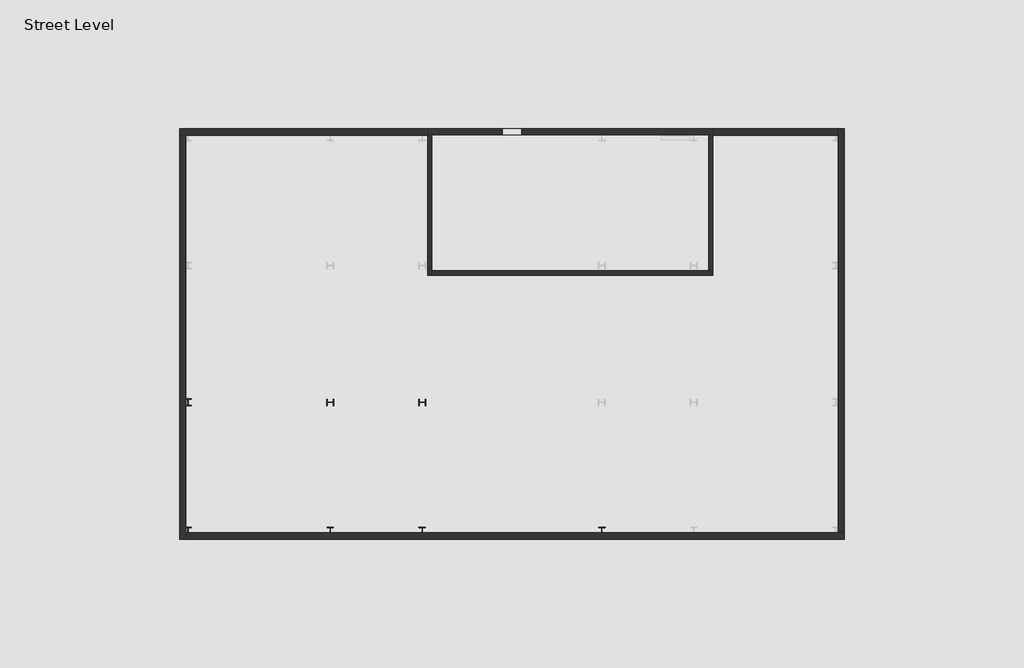
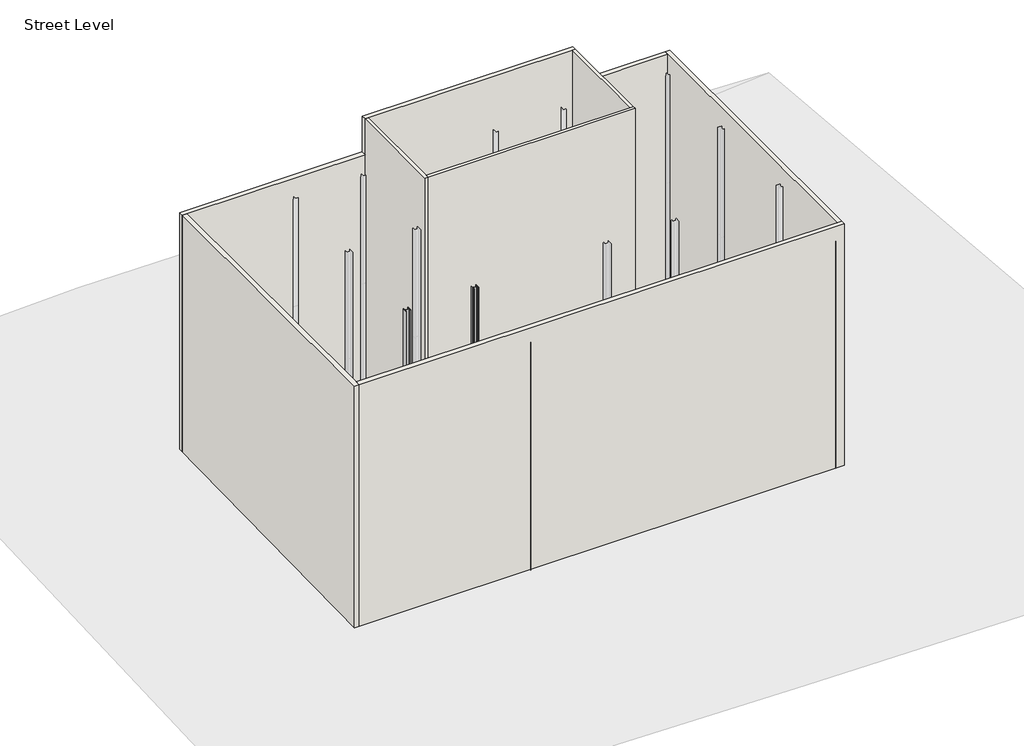
# One storey, part 1 of 3: 9 walls, 7 columns.
"""IFC4 building model written with IfcOpenShell, lengths in millimetres."""

import ifcopenshell
import ifcopenshell.guid

model = None  # the IFC model being written
_history = None  # IfcOwnerHistory: only IFC2X3 demands one
_inside = {}  # id of a spatial element -> (the spatial element, [elements in it])
_under = {}  # id of a project, library or spatial element -> (it, [spatial elements below it])
_declared = {}  # id of a project -> (the project, [libraries it declares])
_typed = {}  # id of a type object -> (the type object, [elements of that type])
_made_of = {}  # id of a material, layer set ... -> (it, [elements and type objects made of it])


def new_model(schema):
    """Start an empty IFC model of exactly this schema.

    Asked for "IFC4X3", IfcOpenShell would pick the latest addendum, in which some entities
    have other attributes; the version numbers below select the first issue.
    IFC2X3 requires an IfcOwnerHistory on every rooted entity: one is made here for all.
    """
    global model, _history
    if schema == "IFC4X3":
        model = ifcopenshell.file(schema_version=(4, 3, 0, 0))
    else:
        model = ifcopenshell.file(schema=schema)
    _inside.clear()
    _under.clear()
    _declared.clear()
    _typed.clear()
    _made_of.clear()
    _history = None
    if model.schema == "IFC2X3":
        org = make("IfcOrganization", Name="unknown")
        user = make(
            "IfcPersonAndOrganization",
            ThePerson=make("IfcPerson", FamilyName="unknown"),
            TheOrganization=org,
        )
        app = make(
            "IfcApplication",
            ApplicationDeveloper=org,
            Version="unknown",
            ApplicationFullName="unknown",
            ApplicationIdentifier="unknown",
        )
        _history = make(
            "IfcOwnerHistory",
            OwningUser=user,
            OwningApplication=app,
            ChangeAction="ADDED",
            CreationDate=0,
        )
    return model


def make(cls, **values):
    """One entity of the class cls with the attributes given. An attribute that is None is left unset."""
    return model.create_entity(
        cls, **{name: value for name, value in values.items() if value is not None}
    )


def rooted(cls, **values):
    """An entity with a GlobalId (a new one), such as an element, a storey or a relation."""
    return make(cls, GlobalId=ifcopenshell.guid.new(), OwnerHistory=_history, **values)


def si_unit(unit_type, name, prefix=None):
    """IfcSIUnit, for example si_unit("LENGTHUNIT", "METRE", prefix="MILLI")."""
    return make("IfcSIUnit", UnitType=unit_type, Prefix=prefix, Name=name)


def assignment(units):
    """IfcUnitAssignment: the units of a project."""
    return None if units is None else make("IfcUnitAssignment", Units=units)


def point(xyz):
    """IfcCartesianPoint."""
    return None if xyz is None else make("IfcCartesianPoint", Coordinates=xyz)


def direction(xyz):
    """IfcDirection."""
    return None if xyz is None else make("IfcDirection", DirectionRatios=xyz)


def frame(location, z_axis=None, x_axis=None):
    """IfcAxis2Placement3D, a coordinate frame: its origin and axes. An axis left out is left unset."""
    return make(
        "IfcAxis2Placement3D",
        Location=point(location),
        Axis=direction(z_axis),
        RefDirection=direction(x_axis),
    )


def frame_2d(location, x_axis=None):
    """IfcAxis2Placement2D, a coordinate frame in the plane: its origin and x axis."""
    return make(
        "IfcAxis2Placement2D", Location=point(location), RefDirection=direction(x_axis)
    )


def origin():
    """The frame at (0, 0, 0) with its axes left unset."""
    return frame((0.0, 0.0, 0.0))


def place(relative_to, where):
    """IfcLocalPlacement: puts the frame where relative to a parent placement (None: the world)."""
    return make(
        "IfcLocalPlacement", PlacementRelTo=relative_to, RelativePlacement=where
    )


def context(
    kind, dimensions, precision=None, world=None, true_north=None, identifier=None
):
    """IfcGeometricRepresentationContext, for example the 3D "Model" context."""
    return make(
        "IfcGeometricRepresentationContext",
        ContextIdentifier=identifier,
        ContextType=kind,
        CoordinateSpaceDimension=dimensions,
        Precision=precision,
        WorldCoordinateSystem=world,
        TrueNorth=true_north,
    )


def project(units=None, contexts=None):
    """IfcProject with its units and contexts."""
    return rooted(
        "IfcProject",
        Name="project",
        RepresentationContexts=contexts,
        UnitsInContext=assignment(units),
    )


def spatial(cls, under=None, at=None, **own):
    """A site, building, storey or space (cls), placed at a placement, below another one or the project."""
    s = rooted(cls, ObjectPlacement=at, **own)
    if under is not None:
        _under.setdefault(under.id(), (under, []))[1].append(s)
    return s


def polyline(points):
    """IfcPolyline through the points."""
    return make("IfcPolyline", Points=[point(p) for p in points])


def circle_curve(where, radius):
    """IfcCircle in the frame where."""
    return make("IfcCircle", Position=where, Radius=radius)


def trimmed(basis, trim1, trim2, sense, master):
    """IfcTrimmedCurve: the piece of a basis curve between two trims."""
    return make(
        "IfcTrimmedCurve",
        BasisCurve=basis,
        Trim1=trim1,
        Trim2=trim2,
        SenseAgreement=sense,
        MasterRepresentation=master,
    )


def segment(curve, same_sense, transition):
    """IfcCompositeCurveSegment."""
    return make(
        "IfcCompositeCurveSegment",
        Transition=transition,
        SameSense=same_sense,
        ParentCurve=curve,
    )


def composite_curve(segments, self_intersect=None):
    """IfcCompositeCurve: segments joined end to end."""
    return make("IfcCompositeCurve", Segments=segments, SelfIntersect=self_intersect)


def outline(outer, holes=None, kind="AREA"):
    """IfcArbitraryClosedProfileDef: a profile drawn as a closed curve; with holes, ...WithVoids."""
    if holes is None:
        return make("IfcArbitraryClosedProfileDef", ProfileType=kind, OuterCurve=outer)
    return make(
        "IfcArbitraryProfileDefWithVoids",
        ProfileType=kind,
        OuterCurve=outer,
        InnerCurves=holes,
    )


def extrude(swept, where, along, depth):
    """IfcExtrudedAreaSolid: the profile swept, set in the frame where, extruded along a direction by depth."""
    return make(
        "IfcExtrudedAreaSolid",
        SweptArea=swept,
        Position=where,
        ExtrudedDirection=direction(along),
        Depth=depth,
    )


def faces_of(points, faces, orient=None, outer=None):
    """IfcFace entities. A face is a list of loops; a loop is a list of indices into points, from 0.

    orient and outer hold one flag for each loop. By default every Orientation is true, the
    first loop of a face is its IfcFaceOuterBound and the others are IfcFaceBound.
    """
    made = []
    for i, loops in enumerate(faces):
        bounds = []
        for j, loop in enumerate(loops):
            is_outer = j == 0 if outer is None else outer[i][j]
            bounds.append(
                make(
                    "IfcFaceOuterBound" if is_outer else "IfcFaceBound",
                    Bound=make("IfcPolyLoop", Polygon=[points[k] for k in loop]),
                    Orientation=True if orient is None else orient[i][j],
                )
            )
        made.append(make("IfcFace", Bounds=bounds))
    return made


def faceted_brep(points, faces, orient=None, outer=None, voids=None):
    """IfcFacetedBrep: a solid bounded by flat faces; with voids (closed shells), ...WithVoids."""
    shared = [point(p) for p in points]
    hull = make("IfcClosedShell", CfsFaces=faces_of(shared, faces, orient, outer))
    if voids is None:
        return make("IfcFacetedBrep", Outer=hull)
    return make(
        "IfcFacetedBrepWithVoids",
        Outer=hull,
        Voids=[
            make(cls, CfsFaces=faces_of(shared, fs, o, b)) for cls, fs, o, b in voids
        ],
    )


def shape(context_of_items, identifier, shape_type, items):
    """IfcShapeRepresentation: the items that make up one representation, for example the "Body"."""
    return make(
        "IfcShapeRepresentation",
        ContextOfItems=context_of_items,
        RepresentationIdentifier=identifier,
        RepresentationType=shape_type,
        Items=items,
    )


def made_of(thing, what):
    """Note that an element or type object is made of a material, layer set ...; save() writes the relation."""
    if what is not None:
        _made_of.setdefault(what.id(), (what, []))[1].append(thing)
    return thing


def element(
    cls,
    number,
    at=None,
    inside=None,
    cuts=None,
    type_object=None,
    material=None,
    context=None,
    identifier="Body",
    shape_type=None,
    held_by="IfcProductDefinitionShape",
    body=None,
    shapes=None,
    **own,
):
    """One element of the class cls, such as IfcWall. Its Tag is "e" and its number.

    at: its placement. inside: the storey or other place that contains it. cuts: it is an
    opening in that element (IfcRelVoidsElement). A single representation is given by context,
    identifier, shape_type and body (its items); several are given by shapes. held_by: the class
    of the entity that holds the representations. save() writes the other relations.
    """
    e = rooted(cls, Tag="e%d" % number, ObjectPlacement=at, **own)
    if body is not None:
        shapes = [shape(context, identifier, shape_type, body)]
    if shapes is not None:
        e.Representation = make(held_by, Representations=shapes)
    if inside is not None:
        _inside.setdefault(inside.id(), (inside, []))[1].append(e)
    if cuts is not None:
        rooted(
            "IfcRelVoidsElement", RelatingBuildingElement=cuts, RelatedOpeningElement=e
        )
    if type_object is not None:
        _typed.setdefault(type_object.id(), (type_object, []))[1].append(e)
    return made_of(e, material)


def aggregate(whole, parts):
    """IfcRelAggregates: a whole, such as a stair, and the parts it consists of."""
    return rooted("IfcRelAggregates", RelatingObject=whole, RelatedObjects=parts)


def save(model, path):
    """Write the relations noted so far, then the file.

    IfcRelAggregates (storeys below a building ...), IfcRelContainedInSpatialStructure (elements
    in a storey), IfcRelDefinesByType, IfcRelAssociatesMaterial and IfcRelDeclares: one each for
    every whole, place, type object, material and project.
    """
    for whole, parts in _under.values():
        aggregate(whole, parts)
    for where, things in _inside.values():
        rooted(
            "IfcRelContainedInSpatialStructure",
            RelatedElements=things,
            RelatingStructure=where,
        )
    for kind, things in _typed.values():
        rooted("IfcRelDefinesByType", RelatedObjects=things, RelatingType=kind)
    for what, things in _made_of.values():
        rooted("IfcRelAssociatesMaterial", RelatedObjects=things, RelatingMaterial=what)
    for by, libraries in _declared.values():
        rooted("IfcRelDeclares", RelatingContext=by, RelatedDefinitions=libraries)
    model.write(path)


model = new_model("IFC4")

# Units and contexts
model_context = context("Model", 3, world=origin())
ifc_project = project(units=[si_unit("LENGTHUNIT", "METRE", prefix="MILLI")], contexts=[model_context])

# Site, building, storey
site = spatial("IfcSite", under=ifc_project)
building = spatial("IfcBuilding", under=site)
storey = spatial("IfcBuildingStorey", under=building, Name="Street Level", Elevation=-914.4)

# Columns
placement = place(None, origin())
element("IfcColumn", 1, ObjectType="W-Wide Flange-Column : W12X87", at=placement, inside=storey, context=model_context, shape_type="SweptSolid", body=[
    extrude(outline(composite_curve([segment(polyline([(-9643.0622732, -3562.1684696), (-9663.6362732, -3562.1684696), (-9663.6362732, -3437.3274696)]), True, "CONTINUOUS"), segment(trimmed(circle_curve(frame_2d((-9685.9247732, -3437.3274696)), 22.2885), [point((-9663.6362732, -3437.3274696))], [point((-9685.9247732, -3415.0389696))], True, "CARTESIAN"), True, "CONTINUOUS"), segment(polyline([(-9685.9247732, -3415.0389696), (-9917.6997732, -3415.0389696)]), True, "CONTINUOUS"), segment(trimmed(circle_curve(frame_2d((-9917.6997732, -3437.3274696)), 22.2885), [point((-9917.6997732, -3415.0389696))], [point((-9939.9882732, -3437.3274696))], True, "CARTESIAN"), True, "CONTINUOUS"), segment(polyline([(-9939.9882732, -3437.3274696), (-9939.9882732, -3562.1684696), (-9960.5622732, -3562.1684696), (-9960.5622732, -3254.8284696), (-9939.9882732, -3254.8284696), (-9939.9882732, -3379.6694696)]), True, "CONTINUOUS"), segment(trimmed(circle_curve(frame_2d((-9917.6997732, -3379.6694696)), 22.2885), [point((-9939.9882732, -3379.6694696))], [point((-9917.6997732, -3401.9579696))], True, "CARTESIAN"), True, "CONTINUOUS"), segment(polyline([(-9917.6997732, -3401.9579696), (-9685.9247732, -3401.9579696)]), True, "CONTINUOUS"), segment(trimmed(circle_curve(frame_2d((-9685.9247732, -3379.6694696)), 22.2885), [point((-9685.9247732, -3401.9579696))], [point((-9663.6362732, -3379.6694696))], True, "CARTESIAN"), True, "CONTINUOUS"), segment(polyline([(-9663.6362732, -3379.6694696), (-9663.6362732, -3254.8284696), (-9643.0622732, -3254.8284696), (-9643.0622732, -3562.1684696)]), True, "CONTINUOUS")], self_intersect=False)), frame((0.0, 0.0, 7315.2), z_axis=(0.0, 0.0, 1.0), x_axis=(1.0, 0.0, 0.0)), (0.0, 0.0, 1.0), 7315.2),
    extrude(outline(composite_curve([segment(polyline([(-9643.0622732, -3562.1684696), (-9663.6362732, -3562.1684696), (-9663.6362732, -3437.3274696)]), True, "CONTINUOUS"), segment(trimmed(circle_curve(frame_2d((-9685.9247732, -3437.3274696)), 22.2885), [point((-9663.6362732, -3437.3274696))], [point((-9685.9247732, -3415.0389696))], True, "CARTESIAN"), True, "CONTINUOUS"), segment(polyline([(-9685.9247732, -3415.0389696), (-9917.6997732, -3415.0389696)]), True, "CONTINUOUS"), segment(trimmed(circle_curve(frame_2d((-9917.6997732, -3437.3274696)), 22.2885), [point((-9917.6997732, -3415.0389696))], [point((-9939.9882732, -3437.3274696))], True, "CARTESIAN"), True, "CONTINUOUS"), segment(polyline([(-9939.9882732, -3437.3274696), (-9939.9882732, -3562.1684696), (-9960.5622732, -3562.1684696), (-9960.5622732, -3254.8284696), (-9939.9882732, -3254.8284696), (-9939.9882732, -3379.6694696)]), True, "CONTINUOUS"), segment(trimmed(circle_curve(frame_2d((-9917.6997732, -3379.6694696)), 22.2885), [point((-9939.9882732, -3379.6694696))], [point((-9917.6997732, -3401.9579696))], True, "CARTESIAN"), True, "CONTINUOUS"), segment(polyline([(-9917.6997732, -3401.9579696), (-9685.9247732, -3401.9579696)]), True, "CONTINUOUS"), segment(trimmed(circle_curve(frame_2d((-9685.9247732, -3379.6694696)), 22.2885), [point((-9685.9247732, -3401.9579696))], [point((-9663.6362732, -3379.6694696))], True, "CARTESIAN"), True, "CONTINUOUS"), segment(polyline([(-9663.6362732, -3379.6694696), (-9663.6362732, -3254.8284696), (-9643.0622732, -3254.8284696), (-9643.0622732, -3562.1684696)]), True, "CONTINUOUS")], self_intersect=False)), frame((0.0, 0.0, -914.4), z_axis=(0.0, 0.0, 1.0), x_axis=(1.0, 0.0, 0.0)), (0.0, 0.0, 1.0), 8229.6),
])
element("IfcColumn", 2, ObjectType="W-Wide Flange-Column : W12X87", at=placement, inside=storey, context=model_context, shape_type="SweptSolid", body=[
    extrude(outline(composite_curve([segment(polyline([(-5274.2622732, -3562.1684696), (-5294.8362732, -3562.1684696), (-5294.8362732, -3437.3274696)]), True, "CONTINUOUS"), segment(trimmed(circle_curve(frame_2d((-5317.1247732, -3437.3274696)), 22.2885), [point((-5294.8362732, -3437.3274696))], [point((-5317.1247732, -3415.0389696))], True, "CARTESIAN"), True, "CONTINUOUS"), segment(polyline([(-5317.1247732, -3415.0389696), (-5548.8997732, -3415.0389696)]), True, "CONTINUOUS"), segment(trimmed(circle_curve(frame_2d((-5548.8997732, -3437.3274696)), 22.2885), [point((-5548.8997732, -3415.0389696))], [point((-5571.1882732, -3437.3274696))], True, "CARTESIAN"), True, "CONTINUOUS"), segment(polyline([(-5571.1882732, -3437.3274696), (-5571.1882732, -3562.1684696), (-5591.7622732, -3562.1684696), (-5591.7622732, -3254.8284696), (-5571.1882732, -3254.8284696), (-5571.1882732, -3379.6694696)]), True, "CONTINUOUS"), segment(trimmed(circle_curve(frame_2d((-5548.8997732, -3379.6694696)), 22.2885), [point((-5571.1882732, -3379.6694696))], [point((-5548.8997732, -3401.9579696))], True, "CARTESIAN"), True, "CONTINUOUS"), segment(polyline([(-5548.8997732, -3401.9579696), (-5317.1247732, -3401.9579696)]), True, "CONTINUOUS"), segment(trimmed(circle_curve(frame_2d((-5317.1247732, -3379.6694696)), 22.2885), [point((-5317.1247732, -3401.9579696))], [point((-5294.8362732, -3379.6694696))], True, "CARTESIAN"), True, "CONTINUOUS"), segment(polyline([(-5294.8362732, -3379.6694696), (-5294.8362732, -3254.8284696), (-5274.2622732, -3254.8284696), (-5274.2622732, -3562.1684696)]), True, "CONTINUOUS")], self_intersect=False)), frame((0.0, 0.0, 7315.2), z_axis=(0.0, 0.0, 1.0), x_axis=(1.0, 0.0, 0.0)), (0.0, 0.0, 1.0), 7315.2),
    extrude(outline(composite_curve([segment(polyline([(-5274.2622732, -3562.1684696), (-5294.8362732, -3562.1684696), (-5294.8362732, -3437.3274696)]), True, "CONTINUOUS"), segment(trimmed(circle_curve(frame_2d((-5317.1247732, -3437.3274696)), 22.2885), [point((-5294.8362732, -3437.3274696))], [point((-5317.1247732, -3415.0389696))], True, "CARTESIAN"), True, "CONTINUOUS"), segment(polyline([(-5317.1247732, -3415.0389696), (-5548.8997732, -3415.0389696)]), True, "CONTINUOUS"), segment(trimmed(circle_curve(frame_2d((-5548.8997732, -3437.3274696)), 22.2885), [point((-5548.8997732, -3415.0389696))], [point((-5571.1882732, -3437.3274696))], True, "CARTESIAN"), True, "CONTINUOUS"), segment(polyline([(-5571.1882732, -3437.3274696), (-5571.1882732, -3562.1684696), (-5591.7622732, -3562.1684696), (-5591.7622732, -3254.8284696), (-5571.1882732, -3254.8284696), (-5571.1882732, -3379.6694696)]), True, "CONTINUOUS"), segment(trimmed(circle_curve(frame_2d((-5548.8997732, -3379.6694696)), 22.2885), [point((-5571.1882732, -3379.6694696))], [point((-5548.8997732, -3401.9579696))], True, "CARTESIAN"), True, "CONTINUOUS"), segment(polyline([(-5548.8997732, -3401.9579696), (-5317.1247732, -3401.9579696)]), True, "CONTINUOUS"), segment(trimmed(circle_curve(frame_2d((-5317.1247732, -3379.6694696)), 22.2885), [point((-5317.1247732, -3401.9579696))], [point((-5294.8362732, -3379.6694696))], True, "CARTESIAN"), True, "CONTINUOUS"), segment(polyline([(-5294.8362732, -3379.6694696), (-5294.8362732, -3254.8284696), (-5274.2622732, -3254.8284696), (-5274.2622732, -3562.1684696)]), True, "CONTINUOUS")], self_intersect=False)), frame((0.0, 0.0, -914.4), z_axis=(0.0, 0.0, 1.0), x_axis=(1.0, 0.0, 0.0)), (0.0, 0.0, 1.0), 8229.6),
])
element("IfcColumn", 3, ObjectType="W-Wide Flange-Column : W12X87", at=placement, inside=storey, context=model_context, shape_type="SweptSolid", body=[
    extrude(outline(composite_curve([segment(polyline([(3255.0577268, -9345.7484696), (3255.0577268, -9366.3224696), (3130.2167268, -9366.3224696)]), True, "CONTINUOUS"), segment(trimmed(circle_curve(frame_2d((3130.2167268, -9388.6109696)), 22.2885), [point((3130.2167268, -9366.3224696))], [point((3107.9282268, -9388.6109696))], True, "CARTESIAN"), True, "CONTINUOUS"), segment(polyline([(3107.9282268, -9388.6109696), (3107.9282268, -9620.3859696)]), True, "CONTINUOUS"), segment(trimmed(circle_curve(frame_2d((3130.2167268, -9620.3859696)), 22.2885), [point((3107.9282268, -9620.3859696))], [point((3130.2167268, -9642.6744696))], True, "CARTESIAN"), True, "CONTINUOUS"), segment(polyline([(3130.2167268, -9642.6744696), (3255.0577268, -9642.6744696), (3255.0577268, -9663.2484696), (2947.7177268, -9663.2484696), (2947.7177268, -9642.6744696), (3072.5587268, -9642.6744696)]), True, "CONTINUOUS"), segment(trimmed(circle_curve(frame_2d((3072.5587268, -9620.3859696)), 22.2885), [point((3072.5587268, -9642.6744696))], [point((3094.8472268, -9620.3859696))], True, "CARTESIAN"), True, "CONTINUOUS"), segment(polyline([(3094.8472268, -9620.3859696), (3094.8472268, -9388.6109696)]), True, "CONTINUOUS"), segment(trimmed(circle_curve(frame_2d((3072.5587268, -9388.6109696)), 22.2885), [point((3094.8472268, -9388.6109696))], [point((3072.5587268, -9366.3224696))], True, "CARTESIAN"), True, "CONTINUOUS"), segment(polyline([(3072.5587268, -9366.3224696), (2947.7177268, -9366.3224696), (2947.7177268, -9345.7484696), (3255.0577268, -9345.7484696)]), True, "CONTINUOUS")], self_intersect=False)), frame((0.0, 0.0, 7315.2), z_axis=(0.0, 0.0, 1.0), x_axis=(1.0, 0.0, 0.0)), (0.0, 0.0, 1.0), 7315.2),
    extrude(outline(composite_curve([segment(polyline([(3255.0577268, -9345.7484696), (3255.0577268, -9366.3224696), (3130.2167268, -9366.3224696)]), True, "CONTINUOUS"), segment(trimmed(circle_curve(frame_2d((3130.2167268, -9388.6109696)), 22.2885), [point((3130.2167268, -9366.3224696))], [point((3107.9282268, -9388.6109696))], True, "CARTESIAN"), True, "CONTINUOUS"), segment(polyline([(3107.9282268, -9388.6109696), (3107.9282268, -9620.3859696)]), True, "CONTINUOUS"), segment(trimmed(circle_curve(frame_2d((3130.2167268, -9620.3859696)), 22.2885), [point((3107.9282268, -9620.3859696))], [point((3130.2167268, -9642.6744696))], True, "CARTESIAN"), True, "CONTINUOUS"), segment(polyline([(3130.2167268, -9642.6744696), (3255.0577268, -9642.6744696), (3255.0577268, -9663.2484696), (2947.7177268, -9663.2484696), (2947.7177268, -9642.6744696), (3072.5587268, -9642.6744696)]), True, "CONTINUOUS"), segment(trimmed(circle_curve(frame_2d((3072.5587268, -9620.3859696)), 22.2885), [point((3072.5587268, -9642.6744696))], [point((3094.8472268, -9620.3859696))], True, "CARTESIAN"), True, "CONTINUOUS"), segment(polyline([(3094.8472268, -9620.3859696), (3094.8472268, -9388.6109696)]), True, "CONTINUOUS"), segment(trimmed(circle_curve(frame_2d((3072.5587268, -9388.6109696)), 22.2885), [point((3094.8472268, -9388.6109696))], [point((3072.5587268, -9366.3224696))], True, "CARTESIAN"), True, "CONTINUOUS"), segment(polyline([(3072.5587268, -9366.3224696), (2947.7177268, -9366.3224696), (2947.7177268, -9345.7484696), (3255.0577268, -9345.7484696)]), True, "CONTINUOUS")], self_intersect=False)), frame((0.0, 0.0, -914.4), z_axis=(0.0, 0.0, 1.0), x_axis=(1.0, 0.0, 0.0)), (0.0, 0.0, 1.0), 8229.6),
])
element("IfcColumn", 4, ObjectType="W-Wide Flange-Column : W12X87", at=placement, inside=storey, context=model_context, shape_type="SweptSolid", body=[
    extrude(outline(composite_curve([segment(polyline([(-5279.3422732, -9345.7484696), (-5279.3422732, -9366.3224696), (-5404.1832732, -9366.3224696)]), True, "CONTINUOUS"), segment(trimmed(circle_curve(frame_2d((-5404.1832732, -9388.6109696)), 22.2885), [point((-5404.1832732, -9366.3224696))], [point((-5426.4717732, -9388.6109696))], True, "CARTESIAN"), True, "CONTINUOUS"), segment(polyline([(-5426.4717732, -9388.6109696), (-5426.4717732, -9620.3859696)]), True, "CONTINUOUS"), segment(trimmed(circle_curve(frame_2d((-5404.1832732, -9620.3859696)), 22.2885), [point((-5426.4717732, -9620.3859696))], [point((-5404.1832732, -9642.6744696))], True, "CARTESIAN"), True, "CONTINUOUS"), segment(polyline([(-5404.1832732, -9642.6744696), (-5279.3422732, -9642.6744696), (-5279.3422732, -9663.2484696), (-5586.6822732, -9663.2484696), (-5586.6822732, -9642.6744696), (-5461.8412732, -9642.6744696)]), True, "CONTINUOUS"), segment(trimmed(circle_curve(frame_2d((-5461.8412732, -9620.3859696)), 22.2885), [point((-5461.8412732, -9642.6744696))], [point((-5439.5527732, -9620.3859696))], True, "CARTESIAN"), True, "CONTINUOUS"), segment(polyline([(-5439.5527732, -9620.3859696), (-5439.5527732, -9388.6109696)]), True, "CONTINUOUS"), segment(trimmed(circle_curve(frame_2d((-5461.8412732, -9388.6109696)), 22.2885), [point((-5439.5527732, -9388.6109696))], [point((-5461.8412732, -9366.3224696))], True, "CARTESIAN"), True, "CONTINUOUS"), segment(polyline([(-5461.8412732, -9366.3224696), (-5586.6822732, -9366.3224696), (-5586.6822732, -9345.7484696), (-5279.3422732, -9345.7484696)]), True, "CONTINUOUS")], self_intersect=False)), frame((0.0, 0.0, 7315.2), z_axis=(0.0, 0.0, 1.0), x_axis=(1.0, 0.0, 0.0)), (0.0, 0.0, 1.0), 7315.2),
    extrude(outline(composite_curve([segment(polyline([(-5279.3422732, -9345.7484696), (-5279.3422732, -9366.3224696), (-5404.1832732, -9366.3224696)]), True, "CONTINUOUS"), segment(trimmed(circle_curve(frame_2d((-5404.1832732, -9388.6109696)), 22.2885), [point((-5404.1832732, -9366.3224696))], [point((-5426.4717732, -9388.6109696))], True, "CARTESIAN"), True, "CONTINUOUS"), segment(polyline([(-5426.4717732, -9388.6109696), (-5426.4717732, -9620.3859696)]), True, "CONTINUOUS"), segment(trimmed(circle_curve(frame_2d((-5404.1832732, -9620.3859696)), 22.2885), [point((-5426.4717732, -9620.3859696))], [point((-5404.1832732, -9642.6744696))], True, "CARTESIAN"), True, "CONTINUOUS"), segment(polyline([(-5404.1832732, -9642.6744696), (-5279.3422732, -9642.6744696), (-5279.3422732, -9663.2484696), (-5586.6822732, -9663.2484696), (-5586.6822732, -9642.6744696), (-5461.8412732, -9642.6744696)]), True, "CONTINUOUS"), segment(trimmed(circle_curve(frame_2d((-5461.8412732, -9620.3859696)), 22.2885), [point((-5461.8412732, -9642.6744696))], [point((-5439.5527732, -9620.3859696))], True, "CARTESIAN"), True, "CONTINUOUS"), segment(polyline([(-5439.5527732, -9620.3859696), (-5439.5527732, -9388.6109696)]), True, "CONTINUOUS"), segment(trimmed(circle_curve(frame_2d((-5461.8412732, -9388.6109696)), 22.2885), [point((-5439.5527732, -9388.6109696))], [point((-5461.8412732, -9366.3224696))], True, "CARTESIAN"), True, "CONTINUOUS"), segment(polyline([(-5461.8412732, -9366.3224696), (-5586.6822732, -9366.3224696), (-5586.6822732, -9345.7484696), (-5279.3422732, -9345.7484696)]), True, "CONTINUOUS")], self_intersect=False)), frame((0.0, 0.0, -914.4), z_axis=(0.0, 0.0, 1.0), x_axis=(1.0, 0.0, 0.0)), (0.0, 0.0, 1.0), 8229.6),
])
element("IfcColumn", 5, ObjectType="W-Wide Flange-Column : W12X87", at=placement, inside=storey, context=model_context, shape_type="SweptSolid", body=[
    extrude(outline(composite_curve([segment(polyline([(-9648.1422732, -9345.7484696), (-9648.1422732, -9366.3224696), (-9772.9832732, -9366.3224696)]), True, "CONTINUOUS"), segment(trimmed(circle_curve(frame_2d((-9772.9832732, -9388.6109696)), 22.2885), [point((-9772.9832732, -9366.3224696))], [point((-9795.2717732, -9388.6109696))], True, "CARTESIAN"), True, "CONTINUOUS"), segment(polyline([(-9795.2717732, -9388.6109696), (-9795.2717732, -9620.3859696)]), True, "CONTINUOUS"), segment(trimmed(circle_curve(frame_2d((-9772.9832732, -9620.3859696)), 22.2885), [point((-9795.2717732, -9620.3859696))], [point((-9772.9832732, -9642.6744696))], True, "CARTESIAN"), True, "CONTINUOUS"), segment(polyline([(-9772.9832732, -9642.6744696), (-9648.1422732, -9642.6744696), (-9648.1422732, -9663.2484696), (-9955.4822732, -9663.2484696), (-9955.4822732, -9642.6744696), (-9830.6412732, -9642.6744696)]), True, "CONTINUOUS"), segment(trimmed(circle_curve(frame_2d((-9830.6412732, -9620.3859696)), 22.2885), [point((-9830.6412732, -9642.6744696))], [point((-9808.3527732, -9620.3859696))], True, "CARTESIAN"), True, "CONTINUOUS"), segment(polyline([(-9808.3527732, -9620.3859696), (-9808.3527732, -9388.6109696)]), True, "CONTINUOUS"), segment(trimmed(circle_curve(frame_2d((-9830.6412732, -9388.6109696)), 22.2885), [point((-9808.3527732, -9388.6109696))], [point((-9830.6412732, -9366.3224696))], True, "CARTESIAN"), True, "CONTINUOUS"), segment(polyline([(-9830.6412732, -9366.3224696), (-9955.4822732, -9366.3224696), (-9955.4822732, -9345.7484696), (-9648.1422732, -9345.7484696)]), True, "CONTINUOUS")], self_intersect=False)), frame((0.0, 0.0, 7315.2), z_axis=(0.0, 0.0, 1.0), x_axis=(1.0, 0.0, 0.0)), (0.0, 0.0, 1.0), 7315.2),
    extrude(outline(composite_curve([segment(polyline([(-9648.1422732, -9345.7484696), (-9648.1422732, -9366.3224696), (-9772.9832732, -9366.3224696)]), True, "CONTINUOUS"), segment(trimmed(circle_curve(frame_2d((-9772.9832732, -9388.6109696)), 22.2885), [point((-9772.9832732, -9366.3224696))], [point((-9795.2717732, -9388.6109696))], True, "CARTESIAN"), True, "CONTINUOUS"), segment(polyline([(-9795.2717732, -9388.6109696), (-9795.2717732, -9620.3859696)]), True, "CONTINUOUS"), segment(trimmed(circle_curve(frame_2d((-9772.9832732, -9620.3859696)), 22.2885), [point((-9795.2717732, -9620.3859696))], [point((-9772.9832732, -9642.6744696))], True, "CARTESIAN"), True, "CONTINUOUS"), segment(polyline([(-9772.9832732, -9642.6744696), (-9648.1422732, -9642.6744696), (-9648.1422732, -9663.2484696), (-9955.4822732, -9663.2484696), (-9955.4822732, -9642.6744696), (-9830.6412732, -9642.6744696)]), True, "CONTINUOUS"), segment(trimmed(circle_curve(frame_2d((-9830.6412732, -9620.3859696)), 22.2885), [point((-9830.6412732, -9642.6744696))], [point((-9808.3527732, -9620.3859696))], True, "CARTESIAN"), True, "CONTINUOUS"), segment(polyline([(-9808.3527732, -9620.3859696), (-9808.3527732, -9388.6109696)]), True, "CONTINUOUS"), segment(trimmed(circle_curve(frame_2d((-9830.6412732, -9388.6109696)), 22.2885), [point((-9808.3527732, -9388.6109696))], [point((-9830.6412732, -9366.3224696))], True, "CARTESIAN"), True, "CONTINUOUS"), segment(polyline([(-9830.6412732, -9366.3224696), (-9955.4822732, -9366.3224696), (-9955.4822732, -9345.7484696), (-9648.1422732, -9345.7484696)]), True, "CONTINUOUS")], self_intersect=False)), frame((0.0, 0.0, -914.4), z_axis=(0.0, 0.0, 1.0), x_axis=(1.0, 0.0, 0.0)), (0.0, 0.0, 1.0), 8229.6),
])
element("IfcColumn", 6, ObjectType="W-Wide Flange-Column : W12X87", at=placement, inside=storey, context=model_context, shape_type="SweptSolid", body=[
    extrude(outline(composite_curve([segment(polyline([(-16404.5422732, -9345.7484696), (-16404.5422732, -9366.3224696), (-16529.3832732, -9366.3224696)]), True, "CONTINUOUS"), segment(trimmed(circle_curve(frame_2d((-16529.3832732, -9388.6109696)), 22.2885), [point((-16529.3832732, -9366.3224696))], [point((-16551.6717732, -9388.6109696))], True, "CARTESIAN"), True, "CONTINUOUS"), segment(polyline([(-16551.6717732, -9388.6109696), (-16551.6717732, -9620.3859696)]), True, "CONTINUOUS"), segment(trimmed(circle_curve(frame_2d((-16529.3832732, -9620.3859696)), 22.2885), [point((-16551.6717732, -9620.3859696))], [point((-16529.3832732, -9642.6744696))], True, "CARTESIAN"), True, "CONTINUOUS"), segment(polyline([(-16529.3832732, -9642.6744696), (-16404.5422732, -9642.6744696), (-16404.5422732, -9663.2484696), (-16711.8822732, -9663.2484696), (-16711.8822732, -9642.6744696), (-16587.0412732, -9642.6744696)]), True, "CONTINUOUS"), segment(trimmed(circle_curve(frame_2d((-16587.0412732, -9620.3859696)), 22.2885), [point((-16587.0412732, -9642.6744696))], [point((-16564.7527732, -9620.3859696))], True, "CARTESIAN"), True, "CONTINUOUS"), segment(polyline([(-16564.7527732, -9620.3859696), (-16564.7527732, -9388.6109696)]), True, "CONTINUOUS"), segment(trimmed(circle_curve(frame_2d((-16587.0412732, -9388.6109696)), 22.2885), [point((-16564.7527732, -9388.6109696))], [point((-16587.0412732, -9366.3224696))], True, "CARTESIAN"), True, "CONTINUOUS"), segment(polyline([(-16587.0412732, -9366.3224696), (-16711.8822732, -9366.3224696), (-16711.8822732, -9345.7484696), (-16404.5422732, -9345.7484696)]), True, "CONTINUOUS")], self_intersect=False)), frame((0.0, 0.0, 7315.2), z_axis=(0.0, 0.0, 1.0), x_axis=(1.0, 0.0, 0.0)), (0.0, 0.0, 1.0), 7315.2),
    extrude(outline(composite_curve([segment(polyline([(-16404.5422732, -9345.7484696), (-16404.5422732, -9366.3224696), (-16529.3832732, -9366.3224696)]), True, "CONTINUOUS"), segment(trimmed(circle_curve(frame_2d((-16529.3832732, -9388.6109696)), 22.2885), [point((-16529.3832732, -9366.3224696))], [point((-16551.6717732, -9388.6109696))], True, "CARTESIAN"), True, "CONTINUOUS"), segment(polyline([(-16551.6717732, -9388.6109696), (-16551.6717732, -9620.3859696)]), True, "CONTINUOUS"), segment(trimmed(circle_curve(frame_2d((-16529.3832732, -9620.3859696)), 22.2885), [point((-16551.6717732, -9620.3859696))], [point((-16529.3832732, -9642.6744696))], True, "CARTESIAN"), True, "CONTINUOUS"), segment(polyline([(-16529.3832732, -9642.6744696), (-16404.5422732, -9642.6744696), (-16404.5422732, -9663.2484696), (-16711.8822732, -9663.2484696), (-16711.8822732, -9642.6744696), (-16587.0412732, -9642.6744696)]), True, "CONTINUOUS"), segment(trimmed(circle_curve(frame_2d((-16587.0412732, -9620.3859696)), 22.2885), [point((-16587.0412732, -9642.6744696))], [point((-16564.7527732, -9620.3859696))], True, "CARTESIAN"), True, "CONTINUOUS"), segment(polyline([(-16564.7527732, -9620.3859696), (-16564.7527732, -9388.6109696)]), True, "CONTINUOUS"), segment(trimmed(circle_curve(frame_2d((-16587.0412732, -9388.6109696)), 22.2885), [point((-16564.7527732, -9388.6109696))], [point((-16587.0412732, -9366.3224696))], True, "CARTESIAN"), True, "CONTINUOUS"), segment(polyline([(-16587.0412732, -9366.3224696), (-16711.8822732, -9366.3224696), (-16711.8822732, -9345.7484696), (-16404.5422732, -9345.7484696)]), True, "CONTINUOUS")], self_intersect=False)), frame((0.0, 0.0, -914.4), z_axis=(0.0, 0.0, 1.0), x_axis=(1.0, 0.0, 0.0)), (0.0, 0.0, 1.0), 8229.6),
])
element("IfcColumn", 7, ObjectType="W-Wide Flange-Column : W12X87", at=placement, inside=storey, context=model_context, shape_type="SweptSolid", body=[
    extrude(outline(composite_curve([segment(polyline([(-16404.5422732, -3249.7484696), (-16404.5422732, -3270.3224696), (-16529.3832732, -3270.3224696)]), True, "CONTINUOUS"), segment(trimmed(circle_curve(frame_2d((-16529.3832732, -3292.6109696)), 22.2885), [point((-16529.3832732, -3270.3224696))], [point((-16551.6717732, -3292.6109696))], True, "CARTESIAN"), True, "CONTINUOUS"), segment(polyline([(-16551.6717732, -3292.6109696), (-16551.6717732, -3524.3859696)]), True, "CONTINUOUS"), segment(trimmed(circle_curve(frame_2d((-16529.3832732, -3524.3859696)), 22.2885), [point((-16551.6717732, -3524.3859696))], [point((-16529.3832732, -3546.6744696))], True, "CARTESIAN"), True, "CONTINUOUS"), segment(polyline([(-16529.3832732, -3546.6744696), (-16404.5422732, -3546.6744696), (-16404.5422732, -3567.2484696), (-16711.8822732, -3567.2484696), (-16711.8822732, -3546.6744696), (-16587.0412732, -3546.6744696)]), True, "CONTINUOUS"), segment(trimmed(circle_curve(frame_2d((-16587.0412732, -3524.3859696)), 22.2885), [point((-16587.0412732, -3546.6744696))], [point((-16564.7527732, -3524.3859696))], True, "CARTESIAN"), True, "CONTINUOUS"), segment(polyline([(-16564.7527732, -3524.3859696), (-16564.7527732, -3292.6109696)]), True, "CONTINUOUS"), segment(trimmed(circle_curve(frame_2d((-16587.0412732, -3292.6109696)), 22.2885), [point((-16564.7527732, -3292.6109696))], [point((-16587.0412732, -3270.3224696))], True, "CARTESIAN"), True, "CONTINUOUS"), segment(polyline([(-16587.0412732, -3270.3224696), (-16711.8822732, -3270.3224696), (-16711.8822732, -3249.7484696), (-16404.5422732, -3249.7484696)]), True, "CONTINUOUS")], self_intersect=False)), frame((0.0, 0.0, 7315.2), z_axis=(0.0, 0.0, 1.0), x_axis=(1.0, 0.0, 0.0)), (0.0, 0.0, 1.0), 7315.2),
    extrude(outline(composite_curve([segment(polyline([(-16404.5422732, -3249.7484696), (-16404.5422732, -3270.3224696), (-16529.3832732, -3270.3224696)]), True, "CONTINUOUS"), segment(trimmed(circle_curve(frame_2d((-16529.3832732, -3292.6109696)), 22.2885), [point((-16529.3832732, -3270.3224696))], [point((-16551.6717732, -3292.6109696))], True, "CARTESIAN"), True, "CONTINUOUS"), segment(polyline([(-16551.6717732, -3292.6109696), (-16551.6717732, -3524.3859696)]), True, "CONTINUOUS"), segment(trimmed(circle_curve(frame_2d((-16529.3832732, -3524.3859696)), 22.2885), [point((-16551.6717732, -3524.3859696))], [point((-16529.3832732, -3546.6744696))], True, "CARTESIAN"), True, "CONTINUOUS"), segment(polyline([(-16529.3832732, -3546.6744696), (-16404.5422732, -3546.6744696), (-16404.5422732, -3567.2484696), (-16711.8822732, -3567.2484696), (-16711.8822732, -3546.6744696), (-16587.0412732, -3546.6744696)]), True, "CONTINUOUS"), segment(trimmed(circle_curve(frame_2d((-16587.0412732, -3524.3859696)), 22.2885), [point((-16587.0412732, -3546.6744696))], [point((-16564.7527732, -3524.3859696))], True, "CARTESIAN"), True, "CONTINUOUS"), segment(polyline([(-16564.7527732, -3524.3859696), (-16564.7527732, -3292.6109696)]), True, "CONTINUOUS"), segment(trimmed(circle_curve(frame_2d((-16587.0412732, -3292.6109696)), 22.2885), [point((-16564.7527732, -3292.6109696))], [point((-16587.0412732, -3270.3224696))], True, "CARTESIAN"), True, "CONTINUOUS"), segment(polyline([(-16587.0412732, -3270.3224696), (-16711.8822732, -3270.3224696), (-16711.8822732, -3249.7484696), (-16404.5422732, -3249.7484696)]), True, "CONTINUOUS")], self_intersect=False)), frame((0.0, 0.0, -914.4), z_axis=(0.0, 0.0, 1.0), x_axis=(1.0, 0.0, 0.0)), (0.0, 0.0, 1.0), 8229.6),
])

# Walls
element("IfcWall", 8, ObjectType="Generic - 12\"", at=placement, inside=storey, context=model_context, shape_type="Brep", body=[
    faceted_brep([(-16964.6122732, 9291.5015304, -914.4), (-16659.8122732, 9291.5015304, -914.4), (-5174.2497732, 9291.5015304, -914.4), (-5174.2497732, 9291.5015304, 0.0), (-5174.2497732, 9291.5015304, 3657.6), (-5174.2497732, 9291.5015304, 7315.2), (-5174.2497732, 9291.5015304, 10972.8), (-5174.2497732, 9291.5015304, 14630.4), (-5174.2497732, 9291.5015304, 15849.6), (-16659.8122732, 9291.5015304, 15849.6), (-16964.6122732, 9291.5015304, 15849.6), (-16964.6122732, 9596.3015304, -914.4), (-16964.6122732, 9596.3015304, 15849.6), (-5174.2497732, 9596.3015304, 15849.6), (-5174.2497732, 9596.3015304, -914.4)], [[[0, 1, 2, 3, 4, 5, 6, 7, 8, 9, 10]], [[11, 12, 13, 14]], [[2, 1, 0, 11, 14]], [[10, 9, 8, 13, 12]], [[0, 10, 12, 11]], [[8, 7, 6, 5, 4, 3, 2, 14, 13]]]),
])
element("IfcWall", 9, ObjectType="Generic - 12\"", at=placement, inside=storey, context=model_context, shape_type="Brep", body=[
    faceted_brep([(-16659.8122732, -9910.8984696, -914.4), (-16659.8122732, -9606.0984696, -914.4), (-16659.8122732, 9291.5015304, -914.4), (-16659.8122732, 9291.5015304, 0.0), (-16659.8122732, 9291.5015304, 3657.6), (-16659.8122732, 9291.5015304, 7010.4), (-16659.8122732, 9291.5015304, 7315.2), (-16659.8122732, 9291.5015304, 10972.8), (-16659.8122732, 9291.5015304, 14630.4), (-16659.8122732, 9291.5015304, 15849.6), (-16659.8122732, -9606.0984696, 15849.6), (-16659.8122732, -9910.8984696, 15849.6), (-16964.6122732, -9910.8984696, -914.4), (-16964.6122732, -9910.8984696, 15849.6), (-16964.6122732, 9291.5015304, 15849.6), (-16964.6122732, 9291.5015304, -914.4)], [[[0, 1, 2, 3, 4, 5, 6, 7, 8, 9, 10, 11]], [[12, 13, 14, 15]], [[2, 1, 0, 12, 15]], [[11, 10, 9, 14, 13]], [[0, 11, 13, 12]], [[9, 8, 7, 6, 5, 4, 3, 2, 15, 14]]]),
])
element("IfcWall", 10, ObjectType="Generic - 12\"", at=placement, inside=storey, context=model_context, shape_type="Brep", body=[
    faceted_brep([(14632.9877268, -9606.0984696, -914.4), (14328.1877268, -9606.0984696, -914.4), (-16659.8122732, -9606.0984696, -914.4), (-16659.8122732, -9606.0984696, 0.0), (-16659.8122732, -9606.0984696, 3657.6), (-16659.8122732, -9606.0984696, 7010.4), (-16659.8122732, -9606.0984696, 7315.2), (-16659.8122732, -9606.0984696, 10972.8), (-16659.8122732, -9606.0984696, 14630.4), (-16659.8122732, -9606.0984696, 15849.6), (14328.1877268, -9606.0984696, 15849.6), (14632.9877268, -9606.0984696, 15849.6), (14632.9877268, -9910.8984696, -914.4), (14632.9877268, -9910.8984696, 15849.6), (-16659.8122732, -9910.8984696, 15849.6), (-16659.8122732, -9910.8984696, -914.4)], [[[0, 1, 2, 3, 4, 5, 6, 7, 8, 9, 10, 11]], [[12, 13, 14, 15]], [[2, 1, 0, 12, 15]], [[11, 10, 9, 14, 13]], [[0, 11, 13, 12]], [[9, 8, 7, 6, 5, 4, 3, 2, 15, 14]]]),
])
element("IfcWall", 11, ObjectType="Generic - 12\"", at=placement, inside=storey, context=model_context, shape_type="Brep", body=[
    faceted_brep([(14328.1877268, 9596.3015304, -914.4), (14328.1877268, 9291.5015304, -914.4), (14328.1877268, -9606.0984696, -914.4), (14328.1877268, -9606.0984696, 0.0), (14328.1877268, -9606.0984696, 3657.6), (14328.1877268, -9606.0984696, 7010.4), (14328.1877268, -9606.0984696, 7315.2), (14328.1877268, -9606.0984696, 10972.8), (14328.1877268, -9606.0984696, 14630.4), (14328.1877268, -9606.0984696, 15849.6), (14328.1877268, 9291.5015304, 15849.6), (14328.1877268, 9596.3015304, 15849.6), (14632.9877268, 9596.3015304, -914.4), (14632.9877268, 9596.3015304, 15849.6), (14632.9877268, -9606.0984696, 15849.6), (14632.9877268, -9606.0984696, -914.4)], [[[0, 1, 2, 3, 4, 5, 6, 7, 8, 9, 10, 11]], [[12, 13, 14, 15]], [[2, 1, 0, 12, 15]], [[11, 10, 9, 14, 13]], [[0, 11, 13, 12]], [[9, 8, 7, 6, 5, 4, 3, 2, 15, 14]]]),
])
element("IfcWall", 12, ObjectType="Generic - 12\"", at=placement, inside=storey, context=model_context, shape_type="SweptSolid", body=[
    extrude(outline(polyline([(14328.1877268, 9291.5015304), (8379.8252268, 9291.5015304), (8379.8252268, 9596.3015304), (14328.1877268, 9596.3015304), (14328.1877268, 9291.5015304)])), frame((0.0, 0.0, -914.4), z_axis=(0.0, 0.0, 1.0), x_axis=(1.0, 0.0, 0.0)), (0.0, 0.0, 1.0), 16764.0),
])
element("IfcWall", 13, ObjectType="Generic - 12\" Masonry", at=placement, inside=storey, context=model_context, shape_type="Brep", body=[
    faceted_brep([(-5174.2497732, 9301.0265304, 18288.0), (-5174.2497732, 9301.0265304, -914.4), (-4980.5747732, 9301.0265304, -914.4), (8186.1502268, 9301.0265304, -914.4), (8379.8252268, 9301.0265304, -914.4), (8379.8252268, 9301.0265304, 18288.0), (8186.1502268, 9301.0265304, 18288.0), (-4980.5747732, 9301.0265304, 18288.0), (-708.6122732, 9301.0265304, 0.0), (-1623.0122732, 9301.0265304, 0.0), (-1623.0122732, 9301.0265304, 2133.6), (-708.6122732, 9301.0265304, 2133.6), (-5174.2497732, 9596.3015304, -914.4), (-5174.2497732, 9596.3015304, 18288.0), (8379.8252268, 9596.3015304, 18288.0), (8379.8252268, 9596.3015304, -914.4), (-708.6122732, 9596.3015304, 0.0), (-708.6122732, 9596.3015304, 2133.6), (-1623.0122732, 9596.3015304, 2133.6), (-1623.0122732, 9596.3015304, 0.0)], [[[0, 1, 2, 3, 4, 5, 6, 7], [8, 9, 10, 11]], [[12, 13, 14, 15], [16, 17, 18, 19]], [[4, 3, 2, 1, 12, 15]], [[0, 7, 6, 5, 14, 13]], [[8, 11, 17, 16]], [[11, 10, 18, 17]], [[10, 9, 19, 18]], [[9, 8, 16, 19]], [[0, 13, 12, 1]], [[4, 15, 14, 5]]]),
])
element("IfcWall", 14, ObjectType="Generic - 8\" Masonry", at=placement, inside=storey, context=model_context, shape_type="Brep", body=[
    faceted_brep([(-5174.2497732, 9301.0265304, 18288.0), (-5174.2497732, 9301.0265304, 14630.4), (-5174.2497732, 9301.0265304, 10972.8), (-5174.2497732, 9301.0265304, 7315.2), (-5174.2497732, 9301.0265304, 3657.6), (-5174.2497732, 9301.0265304, 0.0), (-5174.2497732, 9301.0265304, -914.4), (-5174.2497732, 2641.4640304, -914.4), (-5174.2497732, 2641.4640304, 18288.0), (-4980.5747732, 9301.0265304, -914.4), (-4980.5747732, 9301.0265304, 18288.0), (-4980.5747732, 2835.1390304, 18288.0), (-4980.5747732, 2641.4640304, 18288.0), (-4980.5747732, 2641.4640304, -914.4), (-4980.5747732, 2835.1390304, -914.4)], [[[0, 1, 2, 3, 4, 5, 6, 7, 8]], [[9, 10, 11, 12, 13, 14]], [[7, 6, 9, 14, 13]], [[0, 8, 12, 11, 10]], [[8, 7, 13, 12]], [[0, 10, 9, 6, 5, 4, 3, 2, 1]]]),
])
element("IfcWall", 15, ObjectType="Generic - 8\" Masonry", at=placement, inside=storey, context=model_context, shape_type="Brep", body=[
    faceted_brep([(8379.8252268, 2835.1390304, -914.4), (8186.1502268, 2835.1390304, -914.4), (-4980.5747732, 2835.1390304, -914.4), (-4980.5747732, 2835.1390304, 18288.0), (8186.1502268, 2835.1390304, 18288.0), (8379.8252268, 2835.1390304, 18288.0), (8379.8252268, 2641.4640304, -914.4), (8379.8252268, 2641.4640304, 18288.0), (-4980.5747732, 2641.4640304, 18288.0), (-4980.5747732, 2641.4640304, -914.4)], [[[0, 1, 2, 3, 4, 5]], [[6, 7, 8, 9]], [[2, 1, 0, 6, 9]], [[5, 4, 3, 8, 7]], [[3, 2, 9, 8]], [[0, 5, 7, 6]]]),
])
element("IfcWall", 16, ObjectType="Generic - 8\" Masonry", at=placement, inside=storey, context=model_context, shape_type="SweptSolid", body=[
    extrude(outline(polyline([(8186.1502268, 2835.1390304), (8186.1502268, 9301.0265304), (8379.8252268, 9301.0265304), (8379.8252268, 2835.1390304), (8186.1502268, 2835.1390304)])), frame((0.0, 0.0, -914.4), z_axis=(0.0, 0.0, 1.0), x_axis=(1.0, 0.0, 0.0)), (0.0, 0.0, 1.0), 19202.4),
])

save(model, "model.ifc")

# Revit data of these elements
# Project information
#   Organization Name = "G3B Press"
#   Organization Description = "Paul F. Aubin Cosulting Services, Inc."
#   Building Name = "Revit Essentials for Architecture"
#   Author = "Paul F. Aubin"
#   Author Website = "https://www.paulaubin.com"
#   Copyright = "Copyright © 2020 Paul F Aubin, all rights reserved"
#   Project Issue Date = "8/1/2020"
#   Project Status = "Design Development"
#   Client Name = "Column Grids and Structural Layout"
#   Project Address = "123 State ST\nSuite 301\nChicago, IL 60606"
#   Project Name = "06 Commercial_Complete"
#   Project Number = "2020.04A"
# Grids (mm)
#   "1": line (-22547.601, -9504.498) -> (19277.595, -9504.498)
#   "2": line (-22547.601, -3408.498) -> (19277.595, -3408.498)
#   "3": line (-22547.601, 3093.902) -> (19277.595, 3093.902)
#   "4": line (-22547.601, 9189.902) -> (19277.595, 9189.902)
#   "A": line (-16558.212, 12259.726) -> (-16558.212, -14197.104)
#   "B": line (-9801.812, 12259.726) -> (-9801.812, -14197.104)
#   "C": line (-5433.012, 12259.726) -> (-5433.012, -14197.104)
#   "D": line (3101.388, 12259.726) -> (3101.388, -14197.104)
#   "E": line (7470.188, 12259.726) -> (7470.188, -14197.104)
#   "F": line (14226.588, 12259.726) -> (14226.588, -14197.104)
#   "C.3": line (-2689.812, -15151.11) -> (-2689.812, -5965.346)
#   "C.7": line (358.188, -15151.11) -> (358.188, -5965.346)
# Type "W-Wide Flange-Column : W12X87"
#   Assembly Code = "B10"
#   W = 87
#   bf = 1' - 0.1"
#   d = 1' - 0 1/2"
#   k = 0' - 1 11/16"
#   kr = 0' - 0.8775"
#   tf = 0' - 0.81"
#   tw = 0' - 0.515"
#   A = 0.177778 SF
#   Structural Material [instance default] = Steel ASTM A992
# Type "Generic - 12\""
#   Assembly Code = "B2010"
#   Layers, outside or top first: 1' - 0" no material (function 1)
# Type "Generic - 12\" Masonry"
#   Assembly Code = "B2010"
#   Layers, outside or top first: 0' - 11 5/8" "Concrete Masonry Units" (function 1)
# Type "Generic - 8\" Masonry"
#   Assembly Code = "B2010"
#   Layers, outside or top first: 0' - 7 5/8" "Concrete Masonry Units" (function 1)
# Elements 1, 2, 3, 4, 5, 6, 7 (IfcColumn, "W-Wide Flange-Column : W12X87")
#   Structural Material = Steel ASTM A992
#   Phase Created = New Construction
#   Materials on its faces: "Steel ASTM A992"
# Elements 8, 9, 10, 11, 12 (IfcWall, "Generic - 12\"")
#   Top Offset = 4' - 0"
#   Base Offset = 0' - 0"
#   wall height = 55' - 0"
#   Phase Created = New Construction
#   Base Constraint = Street Level
#   Top Constraint = Roof
#   Materials on its faces: "Default Wall"
# Element 13 (IfcWall, "Generic - 12\" Masonry")
#   Top Offset = 12' - 0"
#   Base Offset = 0' - 0"
#   wall height = 63' - 0"
#   Phase Created = New Construction
#   Base Constraint = Street Level
#   Top Constraint = Roof
#   Materials on its faces: "Concrete Masonry Units"
# Elements 14, 15, 16 (IfcWall, "Generic - 8\" Masonry")
#   Comments = ""
#   Top Offset = 12' - 0"
#   Base Offset = 0' - 0"
#   wall height = 63' - 0"
#   Phase Created = New Construction
#   Base Constraint = Street Level
#   Top Constraint = Roof
#   Materials on its faces: "Concrete Masonry Units"
# Materials
#   "Steel ASTM A992": class "Metal", colour RGB 199 199 199, transparency 0, Description = "Structural steel 50ksi", Cost = 0
#   "Concrete Masonry Units": class "Masonry", colour RGB 227 227 227, transparency 0, Description = "Concrete masonry units", Cost = 0
#   "Default Wall": class "Miscellaneous", colour RGB 128 128 128, transparency 0, Cost = 0
